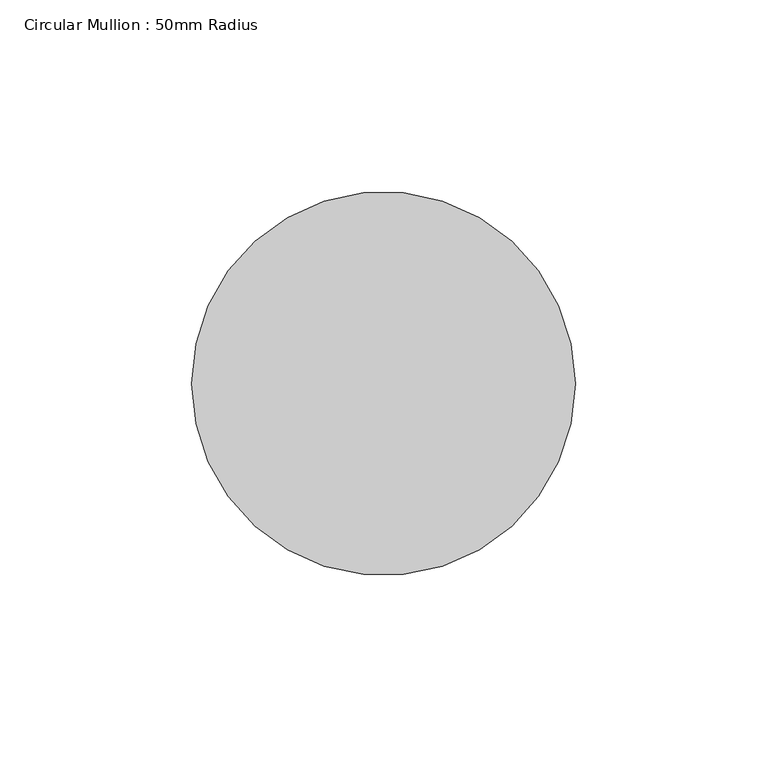
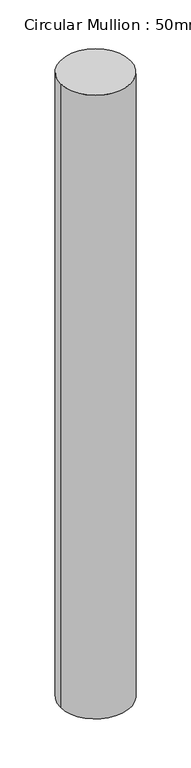
"""IFC4 building model written with IfcOpenShell, lengths in millimetres: member geometry, Circular Mullion : 50mm Radius."""

from ifc_helpers import new_model, si_unit, point, frame, origin, origin_2d, place, context, project, spatial, circle_curve, trimmed, segment, composite_curve, outline, extrude, source, transform, mapped, element, save


def circular_mullion_50mm_radius_c87bddc6(model_context):
    return source(origin(), model_context, "Body", "SweptSolid", [
        extrude(outline(composite_curve([segment(trimmed(circle_curve(origin_2d(), 50.0), [point((50.0, 0.0))], [point((-50.0, 0.0))], False, "CARTESIAN"), True, "CONTINUOUS"), segment(trimmed(circle_curve(origin_2d(), 50.0), [point((-50.0, 0.0))], [point((50.0, 0.0))], False, "CARTESIAN"), True, "CONTINUOUS")], self_intersect=False)), frame((0.0, 0.0, -940.881532), z_axis=(0.0, 0.0, 1.0), x_axis=(1.0, 0.0, 0.0)), (0.0, 0.0, 1.0), 940.881532),
    ])


if __name__ == "__main__":
    model = new_model("IFC4")
    model_context = context("Model", 3, world=origin())
    ifc_project = project(units=[si_unit("LENGTHUNIT", "METRE", prefix="MILLI")], contexts=[model_context])
    site = spatial("IfcSite", under=ifc_project)
    building = spatial("IfcBuilding", under=site)
    placement = place(None, origin())
    circular_mullion_50mm_radius_shape = circular_mullion_50mm_radius_c87bddc6(model_context)
    element("IfcMember", 1, ObjectType="Circular Mullion : 50mm Radius", at=placement, inside=building, context=model_context, shape_type="MappedRepresentation", body=[
        mapped(circular_mullion_50mm_radius_shape, transform((0.0, 0.0, 0.0), x_axis=(1.0, 0.0, 0.0), y_axis=(0.0, 1.0, 0.0), z_axis=(0.0, 0.0, 1.0))),
    ])
    save(model, "model.ifc")

# Revit data of these elements
# Type "Circular Mullion : 50mm Radius"
#   built-in parameter 1007350 = 0.164042 (stored number, unit not read)
# Element 1 (IfcMember, "Circular Mullion : 50mm Radius")
#   Materials on its faces: "Aluminium"
# Materials
#   "Aluminium": class "Metal", colour RGB 247 247 247, transparency 0, Description = "Aluminium 6061", Cost = 0
